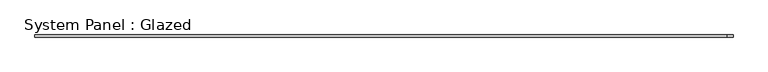
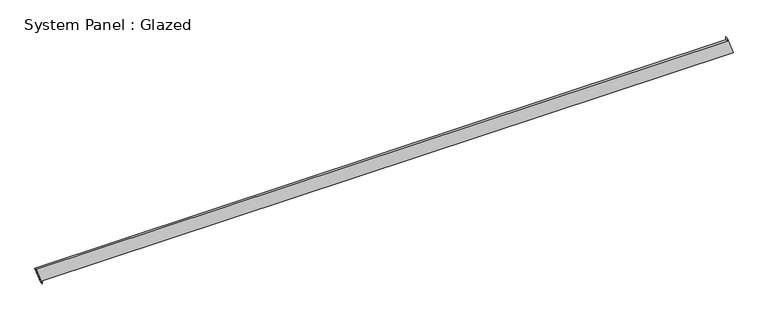
"""IFC4 building model written with IfcOpenShell, lengths in millimetres: plate geometry, System Panel : Glazed."""

import ifcopenshell
import ifcopenshell.guid

model = None  # the IFC model being written
_history = None  # IfcOwnerHistory: only IFC2X3 demands one
_inside = {}  # id of a spatial element -> (the spatial element, [elements in it])
_under = {}  # id of a project, library or spatial element -> (it, [spatial elements below it])
_declared = {}  # id of a project -> (the project, [libraries it declares])
_typed = {}  # id of a type object -> (the type object, [elements of that type])
_made_of = {}  # id of a material, layer set ... -> (it, [elements and type objects made of it])


def new_model(schema):
    """Start an empty IFC model of exactly this schema.

    Asked for "IFC4X3", IfcOpenShell would pick the latest addendum, in which some entities
    have other attributes; the version numbers below select the first issue.
    IFC2X3 requires an IfcOwnerHistory on every rooted entity: one is made here for all.
    """
    global model, _history
    if schema == "IFC4X3":
        model = ifcopenshell.file(schema_version=(4, 3, 0, 0))
    else:
        model = ifcopenshell.file(schema=schema)
    _inside.clear()
    _under.clear()
    _declared.clear()
    _typed.clear()
    _made_of.clear()
    _history = None
    if model.schema == "IFC2X3":
        org = make("IfcOrganization", Name="unknown")
        user = make(
            "IfcPersonAndOrganization",
            ThePerson=make("IfcPerson", FamilyName="unknown"),
            TheOrganization=org,
        )
        app = make(
            "IfcApplication",
            ApplicationDeveloper=org,
            Version="unknown",
            ApplicationFullName="unknown",
            ApplicationIdentifier="unknown",
        )
        _history = make(
            "IfcOwnerHistory",
            OwningUser=user,
            OwningApplication=app,
            ChangeAction="ADDED",
            CreationDate=0,
        )
    return model


def make(cls, **values):
    """One entity of the class cls with the attributes given. An attribute that is None is left unset."""
    return model.create_entity(
        cls, **{name: value for name, value in values.items() if value is not None}
    )


def rooted(cls, **values):
    """An entity with a GlobalId (a new one), such as an element, a storey or a relation."""
    return make(cls, GlobalId=ifcopenshell.guid.new(), OwnerHistory=_history, **values)


def si_unit(unit_type, name, prefix=None):
    """IfcSIUnit, for example si_unit("LENGTHUNIT", "METRE", prefix="MILLI")."""
    return make("IfcSIUnit", UnitType=unit_type, Prefix=prefix, Name=name)


def assignment(units):
    """IfcUnitAssignment: the units of a project."""
    return None if units is None else make("IfcUnitAssignment", Units=units)


def point(xyz):
    """IfcCartesianPoint."""
    return None if xyz is None else make("IfcCartesianPoint", Coordinates=xyz)


def direction(xyz):
    """IfcDirection."""
    return None if xyz is None else make("IfcDirection", DirectionRatios=xyz)


def frame(location, z_axis=None, x_axis=None):
    """IfcAxis2Placement3D, a coordinate frame: its origin and axes. An axis left out is left unset."""
    return make(
        "IfcAxis2Placement3D",
        Location=point(location),
        Axis=direction(z_axis),
        RefDirection=direction(x_axis),
    )


def origin():
    """The frame at (0, 0, 0) with its axes left unset."""
    return frame((0.0, 0.0, 0.0))


def place(relative_to, where):
    """IfcLocalPlacement: puts the frame where relative to a parent placement (None: the world)."""
    return make(
        "IfcLocalPlacement", PlacementRelTo=relative_to, RelativePlacement=where
    )


def context(
    kind, dimensions, precision=None, world=None, true_north=None, identifier=None
):
    """IfcGeometricRepresentationContext, for example the 3D "Model" context."""
    return make(
        "IfcGeometricRepresentationContext",
        ContextIdentifier=identifier,
        ContextType=kind,
        CoordinateSpaceDimension=dimensions,
        Precision=precision,
        WorldCoordinateSystem=world,
        TrueNorth=true_north,
    )


def project(units=None, contexts=None):
    """IfcProject with its units and contexts."""
    return rooted(
        "IfcProject",
        Name="project",
        RepresentationContexts=contexts,
        UnitsInContext=assignment(units),
    )


def spatial(cls, under=None, at=None, **own):
    """A site, building, storey or space (cls), placed at a placement, below another one or the project."""
    s = rooted(cls, ObjectPlacement=at, **own)
    if under is not None:
        _under.setdefault(under.id(), (under, []))[1].append(s)
    return s


def polyline(points):
    """IfcPolyline through the points."""
    return make("IfcPolyline", Points=[point(p) for p in points])


def outline(outer, holes=None, kind="AREA"):
    """IfcArbitraryClosedProfileDef: a profile drawn as a closed curve; with holes, ...WithVoids."""
    if holes is None:
        return make("IfcArbitraryClosedProfileDef", ProfileType=kind, OuterCurve=outer)
    return make(
        "IfcArbitraryProfileDefWithVoids",
        ProfileType=kind,
        OuterCurve=outer,
        InnerCurves=holes,
    )


def extrude(swept, where, along, depth):
    """IfcExtrudedAreaSolid: the profile swept, set in the frame where, extruded along a direction by depth."""
    return make(
        "IfcExtrudedAreaSolid",
        SweptArea=swept,
        Position=where,
        ExtrudedDirection=direction(along),
        Depth=depth,
    )


def shape(context_of_items, identifier, shape_type, items):
    """IfcShapeRepresentation: the items that make up one representation, for example the "Body"."""
    return make(
        "IfcShapeRepresentation",
        ContextOfItems=context_of_items,
        RepresentationIdentifier=identifier,
        RepresentationType=shape_type,
        Items=items,
    )


def source(mapping_origin, context_of_items, identifier, shape_type, items):
    """IfcRepresentationMap: a shape defined once, which mapped items show again and again."""
    return make(
        "IfcRepresentationMap",
        MappingOrigin=mapping_origin,
        MappedRepresentation=shape(context_of_items, identifier, shape_type, items),
    )


def transform(
    local_origin,
    x_axis=None,
    y_axis=None,
    z_axis=None,
    scale=None,
    scale2=None,
    scale3=None,
    uniform=True,
):
    """IfcCartesianTransformationOperator3D, or its non-uniform kind. x_axis, y_axis, z_axis: its Axis1, 2, 3."""
    if uniform:
        return make(
            "IfcCartesianTransformationOperator3D",
            Axis1=direction(x_axis),
            Axis2=direction(y_axis),
            LocalOrigin=point(local_origin),
            Scale=scale,
            Axis3=direction(z_axis),
        )
    return make(
        "IfcCartesianTransformationOperator3DnonUniform",
        Axis1=direction(x_axis),
        Axis2=direction(y_axis),
        LocalOrigin=point(local_origin),
        Scale=scale,
        Axis3=direction(z_axis),
        Scale2=scale2,
        Scale3=scale3,
    )


def mapped(mapping_source, mapping_target):
    """IfcMappedItem: shows the shape of a source again, moved by a transform."""
    return make(
        "IfcMappedItem", MappingSource=mapping_source, MappingTarget=mapping_target
    )


def made_of(thing, what):
    """Note that an element or type object is made of a material, layer set ...; save() writes the relation."""
    if what is not None:
        _made_of.setdefault(what.id(), (what, []))[1].append(thing)
    return thing


def element(
    cls,
    number,
    at=None,
    inside=None,
    cuts=None,
    type_object=None,
    material=None,
    context=None,
    identifier="Body",
    shape_type=None,
    held_by="IfcProductDefinitionShape",
    body=None,
    shapes=None,
    **own,
):
    """One element of the class cls, such as IfcWall. Its Tag is "e" and its number.

    at: its placement. inside: the storey or other place that contains it. cuts: it is an
    opening in that element (IfcRelVoidsElement). A single representation is given by context,
    identifier, shape_type and body (its items); several are given by shapes. held_by: the class
    of the entity that holds the representations. save() writes the other relations.
    """
    e = rooted(cls, Tag="e%d" % number, ObjectPlacement=at, **own)
    if body is not None:
        shapes = [shape(context, identifier, shape_type, body)]
    if shapes is not None:
        e.Representation = make(held_by, Representations=shapes)
    if inside is not None:
        _inside.setdefault(inside.id(), (inside, []))[1].append(e)
    if cuts is not None:
        rooted(
            "IfcRelVoidsElement", RelatingBuildingElement=cuts, RelatedOpeningElement=e
        )
    if type_object is not None:
        _typed.setdefault(type_object.id(), (type_object, []))[1].append(e)
    return made_of(e, material)


def aggregate(whole, parts):
    """IfcRelAggregates: a whole, such as a stair, and the parts it consists of."""
    return rooted("IfcRelAggregates", RelatingObject=whole, RelatedObjects=parts)


def save(model, path):
    """Write the relations noted so far, then the file.

    IfcRelAggregates (storeys below a building ...), IfcRelContainedInSpatialStructure (elements
    in a storey), IfcRelDefinesByType, IfcRelAssociatesMaterial and IfcRelDeclares: one each for
    every whole, place, type object, material and project.
    """
    for whole, parts in _under.values():
        aggregate(whole, parts)
    for where, things in _inside.values():
        rooted(
            "IfcRelContainedInSpatialStructure",
            RelatedElements=things,
            RelatingStructure=where,
        )
    for kind, things in _typed.values():
        rooted("IfcRelDefinesByType", RelatedObjects=things, RelatingType=kind)
    for what, things in _made_of.values():
        rooted("IfcRelAssociatesMaterial", RelatedObjects=things, RelatingMaterial=what)
    for by, libraries in _declared.values():
        rooted("IfcRelDeclares", RelatingContext=by, RelatedDefinitions=libraries)
    model.write(path)


def system_panel_glazed_ea61075c(model_context):
    return source(origin(), model_context, "Body", "SweptSolid", [
        extrude(outline(polyline([(0.0, -3958.7388288), (35.3553391, -3958.7388288), (35.3553391, 4028.1708947), (235.3914127, 3958.6179308), (200.0360737, 3958.6177077), (200.0864778, -4028.1708947), (0.0, -3958.7388288)])), frame((0.0, -49.5, 0.0), z_axis=(0.0, 1.0, 0.0), x_axis=(0.0, 0.0, 1.0)), (0.0, 0.0, 1.0), 25.0),
    ])


if __name__ == "__main__":
    model = new_model("IFC4")
    model_context = context("Model", 3, world=origin())
    ifc_project = project(units=[si_unit("LENGTHUNIT", "METRE", prefix="MILLI")], contexts=[model_context])
    site = spatial("IfcSite", under=ifc_project)
    building = spatial("IfcBuilding", under=site)
    placement = place(None, origin())
    system_panel_glazed_shape = system_panel_glazed_ea61075c(model_context)
    element("IfcPlate", 1, ObjectType="System Panel : Glazed", at=placement, inside=building, context=model_context, shape_type="MappedRepresentation", body=[
        mapped(system_panel_glazed_shape, transform((0.0, 0.0, 0.0), x_axis=(1.0, 0.0, 0.0), y_axis=(0.0, 1.0, 0.0), z_axis=(0.0, 0.0, 1.0))),
    ])
    save(model, "model.ifc")

# Revit data of these elements
# Element 1 (IfcPlate, "System Panel : Glazed")
#   Materials on its faces: "Glass"
# Materials
#   "Glass": class "Glass", colour RGB 218 227 224, transparency 0.85, Description = "Soda Lime Glass", Cost = 0
